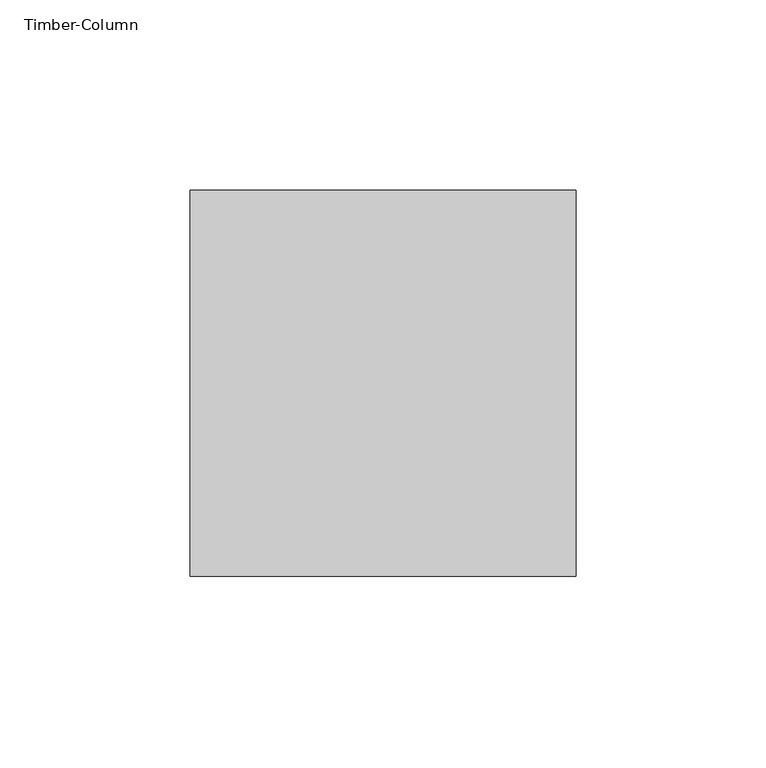
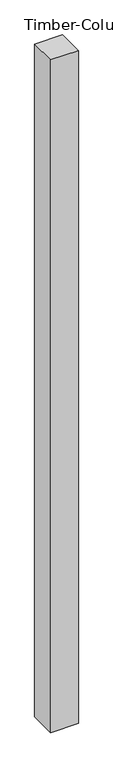
"""IFC4 building model written with IfcOpenShell, lengths in millimetres: column geometry, Timber-Column."""

import ifcopenshell
import ifcopenshell.guid

model = None  # the IFC model being written
_history = None  # IfcOwnerHistory: only IFC2X3 demands one
_inside = {}  # id of a spatial element -> (the spatial element, [elements in it])
_under = {}  # id of a project, library or spatial element -> (it, [spatial elements below it])
_declared = {}  # id of a project -> (the project, [libraries it declares])
_typed = {}  # id of a type object -> (the type object, [elements of that type])
_made_of = {}  # id of a material, layer set ... -> (it, [elements and type objects made of it])


def new_model(schema):
    """Start an empty IFC model of exactly this schema.

    Asked for "IFC4X3", IfcOpenShell would pick the latest addendum, in which some entities
    have other attributes; the version numbers below select the first issue.
    IFC2X3 requires an IfcOwnerHistory on every rooted entity: one is made here for all.
    """
    global model, _history
    if schema == "IFC4X3":
        model = ifcopenshell.file(schema_version=(4, 3, 0, 0))
    else:
        model = ifcopenshell.file(schema=schema)
    _inside.clear()
    _under.clear()
    _declared.clear()
    _typed.clear()
    _made_of.clear()
    _history = None
    if model.schema == "IFC2X3":
        org = make("IfcOrganization", Name="unknown")
        user = make(
            "IfcPersonAndOrganization",
            ThePerson=make("IfcPerson", FamilyName="unknown"),
            TheOrganization=org,
        )
        app = make(
            "IfcApplication",
            ApplicationDeveloper=org,
            Version="unknown",
            ApplicationFullName="unknown",
            ApplicationIdentifier="unknown",
        )
        _history = make(
            "IfcOwnerHistory",
            OwningUser=user,
            OwningApplication=app,
            ChangeAction="ADDED",
            CreationDate=0,
        )
    return model


def make(cls, **values):
    """One entity of the class cls with the attributes given. An attribute that is None is left unset."""
    return model.create_entity(
        cls, **{name: value for name, value in values.items() if value is not None}
    )


def rooted(cls, **values):
    """An entity with a GlobalId (a new one), such as an element, a storey or a relation."""
    return make(cls, GlobalId=ifcopenshell.guid.new(), OwnerHistory=_history, **values)


def si_unit(unit_type, name, prefix=None):
    """IfcSIUnit, for example si_unit("LENGTHUNIT", "METRE", prefix="MILLI")."""
    return make("IfcSIUnit", UnitType=unit_type, Prefix=prefix, Name=name)


def assignment(units):
    """IfcUnitAssignment: the units of a project."""
    return None if units is None else make("IfcUnitAssignment", Units=units)


def point(xyz):
    """IfcCartesianPoint."""
    return None if xyz is None else make("IfcCartesianPoint", Coordinates=xyz)


def direction(xyz):
    """IfcDirection."""
    return None if xyz is None else make("IfcDirection", DirectionRatios=xyz)


def frame(location, z_axis=None, x_axis=None):
    """IfcAxis2Placement3D, a coordinate frame: its origin and axes. An axis left out is left unset."""
    return make(
        "IfcAxis2Placement3D",
        Location=point(location),
        Axis=direction(z_axis),
        RefDirection=direction(x_axis),
    )


def origin():
    """The frame at (0, 0, 0) with its axes left unset."""
    return frame((0.0, 0.0, 0.0))


def place(relative_to, where):
    """IfcLocalPlacement: puts the frame where relative to a parent placement (None: the world)."""
    return make(
        "IfcLocalPlacement", PlacementRelTo=relative_to, RelativePlacement=where
    )


def context(
    kind, dimensions, precision=None, world=None, true_north=None, identifier=None
):
    """IfcGeometricRepresentationContext, for example the 3D "Model" context."""
    return make(
        "IfcGeometricRepresentationContext",
        ContextIdentifier=identifier,
        ContextType=kind,
        CoordinateSpaceDimension=dimensions,
        Precision=precision,
        WorldCoordinateSystem=world,
        TrueNorth=true_north,
    )


def project(units=None, contexts=None):
    """IfcProject with its units and contexts."""
    return rooted(
        "IfcProject",
        Name="project",
        RepresentationContexts=contexts,
        UnitsInContext=assignment(units),
    )


def spatial(cls, under=None, at=None, **own):
    """A site, building, storey or space (cls), placed at a placement, below another one or the project."""
    s = rooted(cls, ObjectPlacement=at, **own)
    if under is not None:
        _under.setdefault(under.id(), (under, []))[1].append(s)
    return s


def polyline(points):
    """IfcPolyline through the points."""
    return make("IfcPolyline", Points=[point(p) for p in points])


def outline(outer, holes=None, kind="AREA"):
    """IfcArbitraryClosedProfileDef: a profile drawn as a closed curve; with holes, ...WithVoids."""
    if holes is None:
        return make("IfcArbitraryClosedProfileDef", ProfileType=kind, OuterCurve=outer)
    return make(
        "IfcArbitraryProfileDefWithVoids",
        ProfileType=kind,
        OuterCurve=outer,
        InnerCurves=holes,
    )


def extrude(swept, where, along, depth):
    """IfcExtrudedAreaSolid: the profile swept, set in the frame where, extruded along a direction by depth."""
    return make(
        "IfcExtrudedAreaSolid",
        SweptArea=swept,
        Position=where,
        ExtrudedDirection=direction(along),
        Depth=depth,
    )


def shape(context_of_items, identifier, shape_type, items):
    """IfcShapeRepresentation: the items that make up one representation, for example the "Body"."""
    return make(
        "IfcShapeRepresentation",
        ContextOfItems=context_of_items,
        RepresentationIdentifier=identifier,
        RepresentationType=shape_type,
        Items=items,
    )


def source(mapping_origin, context_of_items, identifier, shape_type, items):
    """IfcRepresentationMap: a shape defined once, which mapped items show again and again."""
    return make(
        "IfcRepresentationMap",
        MappingOrigin=mapping_origin,
        MappedRepresentation=shape(context_of_items, identifier, shape_type, items),
    )


def transform(
    local_origin,
    x_axis=None,
    y_axis=None,
    z_axis=None,
    scale=None,
    scale2=None,
    scale3=None,
    uniform=True,
):
    """IfcCartesianTransformationOperator3D, or its non-uniform kind. x_axis, y_axis, z_axis: its Axis1, 2, 3."""
    if uniform:
        return make(
            "IfcCartesianTransformationOperator3D",
            Axis1=direction(x_axis),
            Axis2=direction(y_axis),
            LocalOrigin=point(local_origin),
            Scale=scale,
            Axis3=direction(z_axis),
        )
    return make(
        "IfcCartesianTransformationOperator3DnonUniform",
        Axis1=direction(x_axis),
        Axis2=direction(y_axis),
        LocalOrigin=point(local_origin),
        Scale=scale,
        Axis3=direction(z_axis),
        Scale2=scale2,
        Scale3=scale3,
    )


def mapped(mapping_source, mapping_target):
    """IfcMappedItem: shows the shape of a source again, moved by a transform."""
    return make(
        "IfcMappedItem", MappingSource=mapping_source, MappingTarget=mapping_target
    )


def made_of(thing, what):
    """Note that an element or type object is made of a material, layer set ...; save() writes the relation."""
    if what is not None:
        _made_of.setdefault(what.id(), (what, []))[1].append(thing)
    return thing


def element(
    cls,
    number,
    at=None,
    inside=None,
    cuts=None,
    type_object=None,
    material=None,
    context=None,
    identifier="Body",
    shape_type=None,
    held_by="IfcProductDefinitionShape",
    body=None,
    shapes=None,
    **own,
):
    """One element of the class cls, such as IfcWall. Its Tag is "e" and its number.

    at: its placement. inside: the storey or other place that contains it. cuts: it is an
    opening in that element (IfcRelVoidsElement). A single representation is given by context,
    identifier, shape_type and body (its items); several are given by shapes. held_by: the class
    of the entity that holds the representations. save() writes the other relations.
    """
    e = rooted(cls, Tag="e%d" % number, ObjectPlacement=at, **own)
    if body is not None:
        shapes = [shape(context, identifier, shape_type, body)]
    if shapes is not None:
        e.Representation = make(held_by, Representations=shapes)
    if inside is not None:
        _inside.setdefault(inside.id(), (inside, []))[1].append(e)
    if cuts is not None:
        rooted(
            "IfcRelVoidsElement", RelatingBuildingElement=cuts, RelatedOpeningElement=e
        )
    if type_object is not None:
        _typed.setdefault(type_object.id(), (type_object, []))[1].append(e)
    return made_of(e, material)


def aggregate(whole, parts):
    """IfcRelAggregates: a whole, such as a stair, and the parts it consists of."""
    return rooted("IfcRelAggregates", RelatingObject=whole, RelatedObjects=parts)


def save(model, path):
    """Write the relations noted so far, then the file.

    IfcRelAggregates (storeys below a building ...), IfcRelContainedInSpatialStructure (elements
    in a storey), IfcRelDefinesByType, IfcRelAssociatesMaterial and IfcRelDeclares: one each for
    every whole, place, type object, material and project.
    """
    for whole, parts in _under.values():
        aggregate(whole, parts)
    for where, things in _inside.values():
        rooted(
            "IfcRelContainedInSpatialStructure",
            RelatedElements=things,
            RelatingStructure=where,
        )
    for kind, things in _typed.values():
        rooted("IfcRelDefinesByType", RelatedObjects=things, RelatingType=kind)
    for what, things in _made_of.values():
        rooted("IfcRelAssociatesMaterial", RelatedObjects=things, RelatingMaterial=what)
    for by, libraries in _declared.values():
        rooted("IfcRelDeclares", RelatingContext=by, RelatedDefinitions=libraries)
    model.write(path)


def timber_column_b7e6a7b9(model_context):
    return source(origin(), model_context, "Body", "SweptSolid", [
        extrude(outline(polyline([(50.8, 50.8), (50.8, -50.8), (-50.8, -50.8), (-50.8, 50.8), (50.8, 50.8)])), frame((0.0, 0.0, 50.8), z_axis=(0.0, 0.0, 1.0), x_axis=(1.0, 0.0, 0.0)), (0.0, 0.0, 1.0), 2616.2),
    ])


if __name__ == "__main__":
    model = new_model("IFC4")
    model_context = context("Model", 3, world=origin())
    ifc_project = project(units=[si_unit("LENGTHUNIT", "METRE", prefix="MILLI")], contexts=[model_context])
    site = spatial("IfcSite", under=ifc_project)
    building = spatial("IfcBuilding", under=site)
    placement = place(None, origin())
    timber_column_shape = timber_column_b7e6a7b9(model_context)
    element("IfcColumn", 1, ObjectType="Timber-Column : BLDG 6241 Wall Struds 4\"x4\"", at=placement, inside=building, context=model_context, shape_type="MappedRepresentation", body=[
        mapped(timber_column_shape, transform((0.0, 0.0, 0.0), x_axis=(1.0, 0.0, 0.0), y_axis=(0.0, 1.0, 0.0), z_axis=(0.0, 0.0, 1.0))),
    ])
    save(model, "model.ifc")

# Revit data of these elements
# Type "Timber-Column : BLDG 6241 Wall Struds 4\"x4\""
#   Assembly Code = "B10"
#   A = 0.140625 SF
#   b = 0' - 4"
#   d = 0' - 4"
#   Structural Material [instance default] = Softwood, Lumber
# Element 1 (IfcColumn, "Timber-Column : BLDG 6241 Wall Struds 4\"x4\"")
#   Materials on its faces: "Softwood, Lumber"
# Materials
#   "Softwood, Lumber": class "Wood", colour RGB 223 192 134, transparency 0, Description = "Pinus Echinata", Cost = 0
